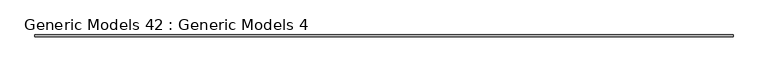
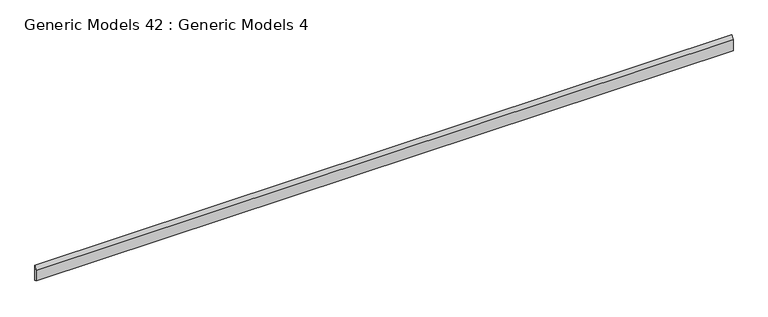
"""IFC4 building model written with IfcOpenShell, lengths in millimetres: proxy geometry, Generic Models 42 : Generic Models 4."""

from ifc_helpers import new_model, si_unit, frame, origin, place, context, project, spatial, polyline, outline, extrude, source, transform, mapped, element, save


def generic_models_42_generic_models_4_13d7cb58(model_context):
    return source(origin(), model_context, "Body", "SweptSolid", [
        extrude(outline(polyline([(14261.3425835, 127006.935011), (14261.3425835, 127109.3314334), (14279.1225835, 127143.9556439), (14279.1225835, 127001.220011), (14261.3425835, 127006.935011)])), frame((-8338.9298025, 0.0, 0.0), z_axis=(1.0, 0.0, 0.0), x_axis=(0.0, 1.0, 0.0)), (0.0, 0.0, 1.0), 6186.756498),
    ])


if __name__ == "__main__":
    model = new_model("IFC4")
    model_context = context("Model", 3, world=origin())
    ifc_project = project(units=[si_unit("LENGTHUNIT", "METRE", prefix="MILLI")], contexts=[model_context])
    site = spatial("IfcSite", under=ifc_project)
    building = spatial("IfcBuilding", under=site)
    placement = place(None, origin())
    generic_models_42_generic_models_4_shape = generic_models_42_generic_models_4_13d7cb58(model_context)
    element("IfcBuildingElementProxy", 1, Name="Generic Models 42 : Generic Models 4", ObjectType="Generic Models 42 : Generic Models 4", at=placement, inside=building, context=model_context, shape_type="MappedRepresentation", body=[
        mapped(generic_models_42_generic_models_4_shape, transform((0.0, 0.0, 0.0), x_axis=(1.0, 0.0, 0.0), y_axis=(0.0, 1.0, 0.0), z_axis=(0.0, 0.0, 1.0))),
    ])
    save(model, "model.ifc")

# Revit data of these elements
# Element 1 (IfcBuildingElementProxy, "Generic Models 42 : Generic Models 4")
#   Materials on its faces: "_7/8\" SMOOTH TROWEL EXTERIOR STUCCO (COLOR PER OWNER)"
# Materials
#   "_7/8\" SMOOTH TROWEL EXTERIOR STUCCO (COLOR PER OWNER)": class "Generic", colour RGB 233 233 233, transparency 0, Cost = 0
